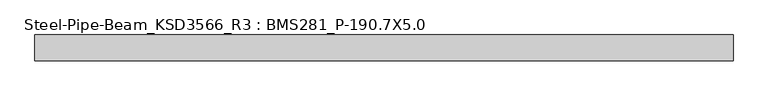
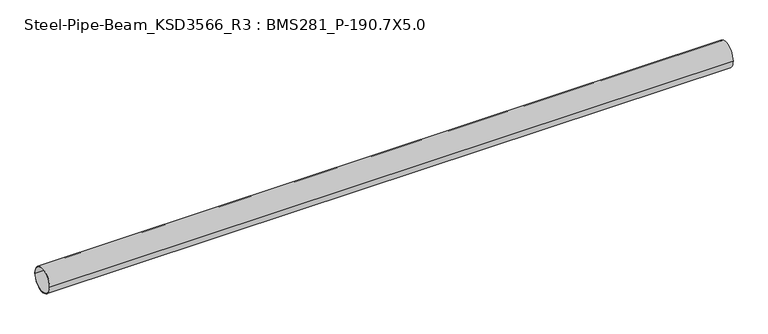
"""IFC4 building model written with IfcOpenShell, lengths in millimetres: member geometry, Steel-Pipe-Beam_KSD3566_R3 : BMS281_P-190.7X5.0."""

from ifc_helpers import new_model, si_unit, point, frame, origin, origin_2d, place, context, project, spatial, circle_curve, trimmed, segment, composite_curve, outline, extrude, source, transform, mapped, element, save


def steel_pipe_beam_ksd3566_r3_bms281_p_190_7x5_0_949b0d8a(model_context):
    return source(origin(), model_context, "Body", "SweptSolid", [
        extrude(outline(composite_curve([segment(trimmed(circle_curve(origin_2d(), 95.35), [point((-95.35, 0.0))], [point((95.35, 0.0))], False, "CARTESIAN"), True, "CONTINUOUS"), segment(trimmed(circle_curve(origin_2d(), 95.35), [point((95.35, 0.0))], [point((-95.35, 0.0))], False, "CARTESIAN"), True, "CONTINUOUS")], self_intersect=False), holes=[composite_curve([segment(trimmed(circle_curve(origin_2d(), 90.35), [point((90.35, 0.0))], [point((-90.35, 0.0))], True, "CARTESIAN"), True, "CONTINUOUS"), segment(trimmed(circle_curve(origin_2d(), 90.35), [point((-90.35, 0.0))], [point((90.35, 0.0))], True, "CARTESIAN"), True, "CONTINUOUS")], self_intersect=False)]), frame((-2587.7859949, 0.0, 0.0), z_axis=(1.0, 0.0, 0.0), x_axis=(0.0, 1.0, 0.0)), (0.0, 0.0, 1.0), 5164.9165514),
    ])


if __name__ == "__main__":
    model = new_model("IFC4")
    model_context = context("Model", 3, world=origin())
    ifc_project = project(units=[si_unit("LENGTHUNIT", "METRE", prefix="MILLI")], contexts=[model_context])
    site = spatial("IfcSite", under=ifc_project)
    building = spatial("IfcBuilding", under=site)
    placement = place(None, origin())
    steel_pipe_beam_ksd3566_r3_bms281_p_190_7x5_0_shape = steel_pipe_beam_ksd3566_r3_bms281_p_190_7x5_0_949b0d8a(model_context)
    element("IfcMember", 1, ObjectType="Steel-Pipe-Beam_KSD3566_R3 : BMS281_P-190.7X5.0", at=placement, inside=building, context=model_context, shape_type="MappedRepresentation", body=[
        mapped(steel_pipe_beam_ksd3566_r3_bms281_p_190_7x5_0_shape, transform((0.0, 0.0, 0.0), x_axis=(1.0, 0.0, 0.0), y_axis=(0.0, 1.0, 0.0), z_axis=(0.0, 0.0, 1.0))),
    ])
    save(model, "model.ifc")

# Revit data of these elements
# Type "Steel-Pipe-Beam_KSD3566_R3 : BMS281_P-190.7X5.0"
#   Keynote = "P-190.7X5.0"
#   SteelWeight = "Light"
#   t = 0.0050 m
#   Surface Area = 0.599102 m²/m
#   Section Area = 29.1697 cm²
#   Mass per Unit Length = 22.8982 kg/m
#   Length [instance default] = 1.5000 m
#   D = 0.1907 m
#   hec_material4 [instance default] = none
#   hec_material3 [instance default] = none
#   hec_material2 [instance default] = none
#   hec_material1 [instance default] = none
#   Structural Material [instance default] = Steel, 45-345
#   Assembly Code = ""
# Element 1 (IfcMember, "Steel-Pipe-Beam_KSD3566_R3 : BMS281_P-190.7X5.0")
#   Structural Material = none
# Materials
#   "Steel, 45-345": class "Metal", colour RGB 189 187 185, transparency 0, Description = "Steel 345 MPa", Cost = 0
